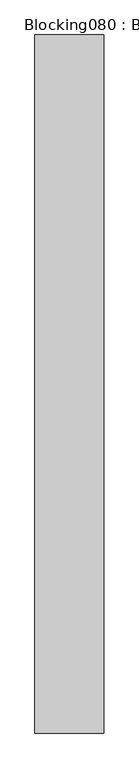
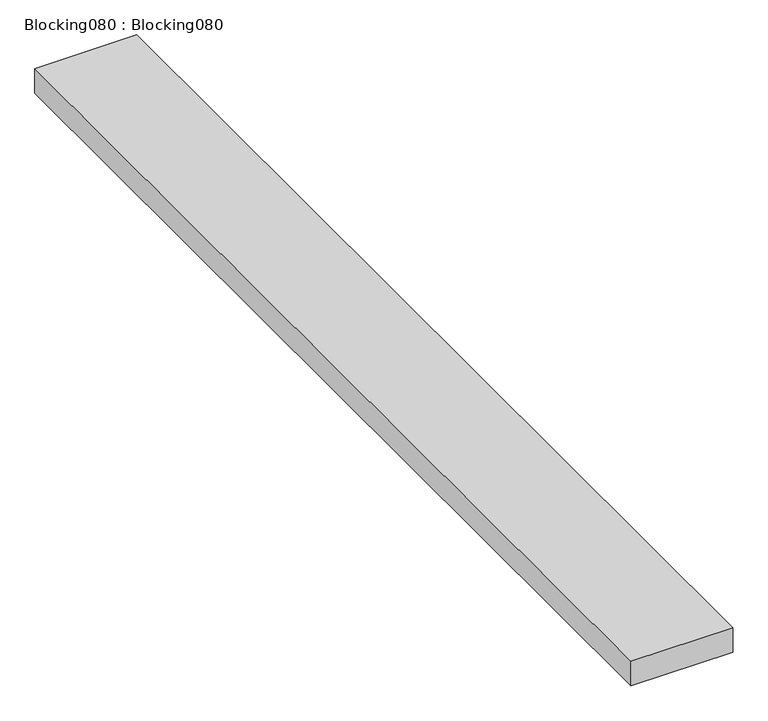
"""IFC4 building model written with IfcOpenShell, lengths in millimetres: proxy geometry, Blocking080 : Blocking080."""

import ifcopenshell
import ifcopenshell.guid

model = None  # the IFC model being written
_history = None  # IfcOwnerHistory: only IFC2X3 demands one
_inside = {}  # id of a spatial element -> (the spatial element, [elements in it])
_under = {}  # id of a project, library or spatial element -> (it, [spatial elements below it])
_declared = {}  # id of a project -> (the project, [libraries it declares])
_typed = {}  # id of a type object -> (the type object, [elements of that type])
_made_of = {}  # id of a material, layer set ... -> (it, [elements and type objects made of it])


def new_model(schema):
    """Start an empty IFC model of exactly this schema.

    Asked for "IFC4X3", IfcOpenShell would pick the latest addendum, in which some entities
    have other attributes; the version numbers below select the first issue.
    IFC2X3 requires an IfcOwnerHistory on every rooted entity: one is made here for all.
    """
    global model, _history
    if schema == "IFC4X3":
        model = ifcopenshell.file(schema_version=(4, 3, 0, 0))
    else:
        model = ifcopenshell.file(schema=schema)
    _inside.clear()
    _under.clear()
    _declared.clear()
    _typed.clear()
    _made_of.clear()
    _history = None
    if model.schema == "IFC2X3":
        org = make("IfcOrganization", Name="unknown")
        user = make(
            "IfcPersonAndOrganization",
            ThePerson=make("IfcPerson", FamilyName="unknown"),
            TheOrganization=org,
        )
        app = make(
            "IfcApplication",
            ApplicationDeveloper=org,
            Version="unknown",
            ApplicationFullName="unknown",
            ApplicationIdentifier="unknown",
        )
        _history = make(
            "IfcOwnerHistory",
            OwningUser=user,
            OwningApplication=app,
            ChangeAction="ADDED",
            CreationDate=0,
        )
    return model


def make(cls, **values):
    """One entity of the class cls with the attributes given. An attribute that is None is left unset."""
    return model.create_entity(
        cls, **{name: value for name, value in values.items() if value is not None}
    )


def rooted(cls, **values):
    """An entity with a GlobalId (a new one), such as an element, a storey or a relation."""
    return make(cls, GlobalId=ifcopenshell.guid.new(), OwnerHistory=_history, **values)


def si_unit(unit_type, name, prefix=None):
    """IfcSIUnit, for example si_unit("LENGTHUNIT", "METRE", prefix="MILLI")."""
    return make("IfcSIUnit", UnitType=unit_type, Prefix=prefix, Name=name)


def assignment(units):
    """IfcUnitAssignment: the units of a project."""
    return None if units is None else make("IfcUnitAssignment", Units=units)


def point(xyz):
    """IfcCartesianPoint."""
    return None if xyz is None else make("IfcCartesianPoint", Coordinates=xyz)


def direction(xyz):
    """IfcDirection."""
    return None if xyz is None else make("IfcDirection", DirectionRatios=xyz)


def frame(location, z_axis=None, x_axis=None):
    """IfcAxis2Placement3D, a coordinate frame: its origin and axes. An axis left out is left unset."""
    return make(
        "IfcAxis2Placement3D",
        Location=point(location),
        Axis=direction(z_axis),
        RefDirection=direction(x_axis),
    )


def origin():
    """The frame at (0, 0, 0) with its axes left unset."""
    return frame((0.0, 0.0, 0.0))


def place(relative_to, where):
    """IfcLocalPlacement: puts the frame where relative to a parent placement (None: the world)."""
    return make(
        "IfcLocalPlacement", PlacementRelTo=relative_to, RelativePlacement=where
    )


def context(
    kind, dimensions, precision=None, world=None, true_north=None, identifier=None
):
    """IfcGeometricRepresentationContext, for example the 3D "Model" context."""
    return make(
        "IfcGeometricRepresentationContext",
        ContextIdentifier=identifier,
        ContextType=kind,
        CoordinateSpaceDimension=dimensions,
        Precision=precision,
        WorldCoordinateSystem=world,
        TrueNorth=true_north,
    )


def project(units=None, contexts=None):
    """IfcProject with its units and contexts."""
    return rooted(
        "IfcProject",
        Name="project",
        RepresentationContexts=contexts,
        UnitsInContext=assignment(units),
    )


def spatial(cls, under=None, at=None, **own):
    """A site, building, storey or space (cls), placed at a placement, below another one or the project."""
    s = rooted(cls, ObjectPlacement=at, **own)
    if under is not None:
        _under.setdefault(under.id(), (under, []))[1].append(s)
    return s


def polyline(points):
    """IfcPolyline through the points."""
    return make("IfcPolyline", Points=[point(p) for p in points])


def outline(outer, holes=None, kind="AREA"):
    """IfcArbitraryClosedProfileDef: a profile drawn as a closed curve; with holes, ...WithVoids."""
    if holes is None:
        return make("IfcArbitraryClosedProfileDef", ProfileType=kind, OuterCurve=outer)
    return make(
        "IfcArbitraryProfileDefWithVoids",
        ProfileType=kind,
        OuterCurve=outer,
        InnerCurves=holes,
    )


def extrude(swept, where, along, depth):
    """IfcExtrudedAreaSolid: the profile swept, set in the frame where, extruded along a direction by depth."""
    return make(
        "IfcExtrudedAreaSolid",
        SweptArea=swept,
        Position=where,
        ExtrudedDirection=direction(along),
        Depth=depth,
    )


def shape(context_of_items, identifier, shape_type, items):
    """IfcShapeRepresentation: the items that make up one representation, for example the "Body"."""
    return make(
        "IfcShapeRepresentation",
        ContextOfItems=context_of_items,
        RepresentationIdentifier=identifier,
        RepresentationType=shape_type,
        Items=items,
    )


def source(mapping_origin, context_of_items, identifier, shape_type, items):
    """IfcRepresentationMap: a shape defined once, which mapped items show again and again."""
    return make(
        "IfcRepresentationMap",
        MappingOrigin=mapping_origin,
        MappedRepresentation=shape(context_of_items, identifier, shape_type, items),
    )


def transform(
    local_origin,
    x_axis=None,
    y_axis=None,
    z_axis=None,
    scale=None,
    scale2=None,
    scale3=None,
    uniform=True,
):
    """IfcCartesianTransformationOperator3D, or its non-uniform kind. x_axis, y_axis, z_axis: its Axis1, 2, 3."""
    if uniform:
        return make(
            "IfcCartesianTransformationOperator3D",
            Axis1=direction(x_axis),
            Axis2=direction(y_axis),
            LocalOrigin=point(local_origin),
            Scale=scale,
            Axis3=direction(z_axis),
        )
    return make(
        "IfcCartesianTransformationOperator3DnonUniform",
        Axis1=direction(x_axis),
        Axis2=direction(y_axis),
        LocalOrigin=point(local_origin),
        Scale=scale,
        Axis3=direction(z_axis),
        Scale2=scale2,
        Scale3=scale3,
    )


def mapped(mapping_source, mapping_target):
    """IfcMappedItem: shows the shape of a source again, moved by a transform."""
    return make(
        "IfcMappedItem", MappingSource=mapping_source, MappingTarget=mapping_target
    )


def made_of(thing, what):
    """Note that an element or type object is made of a material, layer set ...; save() writes the relation."""
    if what is not None:
        _made_of.setdefault(what.id(), (what, []))[1].append(thing)
    return thing


def element(
    cls,
    number,
    at=None,
    inside=None,
    cuts=None,
    type_object=None,
    material=None,
    context=None,
    identifier="Body",
    shape_type=None,
    held_by="IfcProductDefinitionShape",
    body=None,
    shapes=None,
    **own,
):
    """One element of the class cls, such as IfcWall. Its Tag is "e" and its number.

    at: its placement. inside: the storey or other place that contains it. cuts: it is an
    opening in that element (IfcRelVoidsElement). A single representation is given by context,
    identifier, shape_type and body (its items); several are given by shapes. held_by: the class
    of the entity that holds the representations. save() writes the other relations.
    """
    e = rooted(cls, Tag="e%d" % number, ObjectPlacement=at, **own)
    if body is not None:
        shapes = [shape(context, identifier, shape_type, body)]
    if shapes is not None:
        e.Representation = make(held_by, Representations=shapes)
    if inside is not None:
        _inside.setdefault(inside.id(), (inside, []))[1].append(e)
    if cuts is not None:
        rooted(
            "IfcRelVoidsElement", RelatingBuildingElement=cuts, RelatedOpeningElement=e
        )
    if type_object is not None:
        _typed.setdefault(type_object.id(), (type_object, []))[1].append(e)
    return made_of(e, material)


def aggregate(whole, parts):
    """IfcRelAggregates: a whole, such as a stair, and the parts it consists of."""
    return rooted("IfcRelAggregates", RelatingObject=whole, RelatedObjects=parts)


def save(model, path):
    """Write the relations noted so far, then the file.

    IfcRelAggregates (storeys below a building ...), IfcRelContainedInSpatialStructure (elements
    in a storey), IfcRelDefinesByType, IfcRelAssociatesMaterial and IfcRelDeclares: one each for
    every whole, place, type object, material and project.
    """
    for whole, parts in _under.values():
        aggregate(whole, parts)
    for where, things in _inside.values():
        rooted(
            "IfcRelContainedInSpatialStructure",
            RelatedElements=things,
            RelatingStructure=where,
        )
    for kind, things in _typed.values():
        rooted("IfcRelDefinesByType", RelatedObjects=things, RelatingType=kind)
    for what, things in _made_of.values():
        rooted("IfcRelAssociatesMaterial", RelatedObjects=things, RelatingMaterial=what)
    for by, libraries in _declared.values():
        rooted("IfcRelDeclares", RelatingContext=by, RelatedDefinitions=libraries)
    model.write(path)


def blocking080_blocking080_fadc4ae1(model_context):
    return source(origin(), model_context, "Body", "SweptSolid", [
        extrude(outline(polyline([(-4601.0538825, 934.6593428), (-4404.2038825, 934.6593428), (-4404.2038825, -1065.3406572), (-4601.0538825, -1065.3406572), (-4601.0538825, 934.6593428)])), frame((0.0, 0.0, 40182.546), z_axis=(0.0, 0.0, 1.0), x_axis=(1.0, 0.0, 0.0)), (0.0, 0.0, 1.0), 50.8),
    ])


if __name__ == "__main__":
    model = new_model("IFC4")
    model_context = context("Model", 3, world=origin())
    ifc_project = project(units=[si_unit("LENGTHUNIT", "METRE", prefix="MILLI")], contexts=[model_context])
    site = spatial("IfcSite", under=ifc_project)
    building = spatial("IfcBuilding", under=site)
    placement = place(None, origin())
    blocking080_blocking080_shape = blocking080_blocking080_fadc4ae1(model_context)
    element("IfcBuildingElementProxy", 1, Name="Blocking080 : Blocking080", ObjectType="Blocking080 : Blocking080", at=placement, inside=building, context=model_context, shape_type="MappedRepresentation", body=[
        mapped(blocking080_blocking080_shape, transform((0.0, 0.0, 0.0), x_axis=(1.0, 0.0, 0.0), y_axis=(0.0, 1.0, 0.0), z_axis=(0.0, 0.0, 1.0))),
    ])
    save(model, "model.ifc")

# Revit data of these elements
# Type "Blocking080 : Blocking080"
#   NameOverride = "Blocking080"
# Element 1 (IfcBuildingElementProxy, "Blocking080 : Blocking080")
#   Materials on its faces: "WOOD BLOCKING AS REQUIRED"
# Materials
#   "WOOD BLOCKING AS REQUIRED": class "Unassigned", colour RGB 166 124 85, transparency 0, Cost = 0
